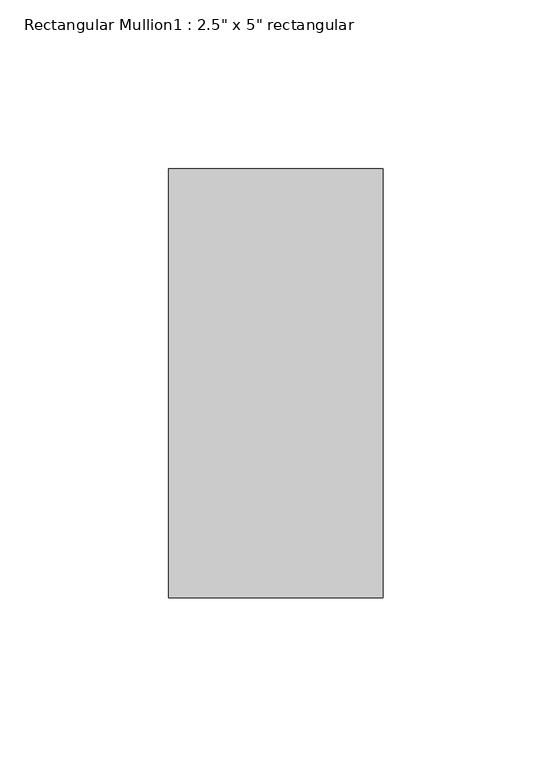
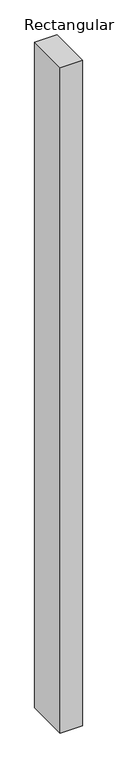
"""IFC4 building model written with IfcOpenShell, lengths in millimetres: member geometry."""

from ifc_helpers import new_model, si_unit, frame, origin, place, context, project, spatial, polyline, outline, extrude, source, transform, mapped, element, save


def member_5e46efc9(model_context):
    return source(origin(), model_context, "Body", "SweptSolid", [
        extrude(outline(polyline([(31.75, 63.5), (31.75, -63.5), (-31.75, -63.5), (-31.75, 63.5), (31.75, 63.5)])), frame((0.0, 0.0, -2021.4166667), z_axis=(0.0, 0.0, 1.0), x_axis=(1.0, 0.0, 0.0)), (0.0, 0.0, 1.0), 2021.4166667),
    ])


if __name__ == "__main__":
    model = new_model("IFC4")
    model_context = context("Model", 3, world=origin())
    ifc_project = project(units=[si_unit("LENGTHUNIT", "METRE", prefix="MILLI")], contexts=[model_context])
    site = spatial("IfcSite", under=ifc_project)
    building = spatial("IfcBuilding", under=site)
    placement = place(None, origin())
    member_shape = member_5e46efc9(model_context)
    element("IfcMember", 1, ObjectType="Rectangular Mullion1 : 2.5\" x 5\" rectangular", at=placement, inside=building, context=model_context, shape_type="MappedRepresentation", body=[
        mapped(member_shape, transform((0.0, 0.0, 0.0), x_axis=(1.0, 0.0, 0.0), y_axis=(0.0, 1.0, 0.0), z_axis=(0.0, 0.0, 1.0))),
    ])
    save(model, "model.ifc")

# Revit data of these elements
# Type "Rectangular Mullion1 : 2.5\" x 5\" rectangular"
#   built-in parameter 1007304 = 0.416667 (stored number, unit not read)
#   built-in parameter 1007301 = 0.104167 (stored number, unit not read)
#   built-in parameter 1007300 = 0.104167 (stored number, unit not read)
# Element 1 (IfcMember, "Rectangular Mullion1 : 2.5\" x 5\" rectangular")
#   Materials on its faces: "support-frame"
# Materials
#   "support-frame": class "Unassigned", colour RGB 233 233 233, transparency 0, Cost = 0
